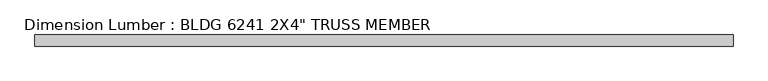
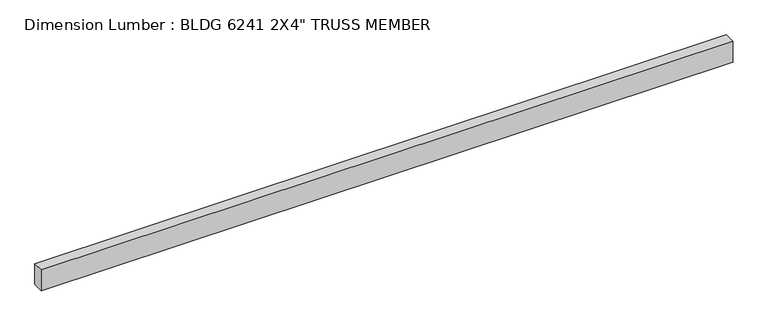
"""IFC4 building model written with IfcOpenShell, lengths in millimetres: beam geometry."""

from ifc_helpers import new_model, si_unit, frame, origin, place, context, project, spatial, polyline, outline, extrude, source, transform, mapped, element, save


def beam_6a2c9f8f(model_context):
    return source(origin(), model_context, "Body", "SweptSolid", [
        extrude(outline(polyline([(1599.9543138, 25.4), (1599.9543138, -25.4), (-1584.2465686, -25.4), (-1584.2465686, 25.4), (1599.9543138, 25.4)])), frame((0.0, 0.0, -50.8), z_axis=(0.0, 0.0, 1.0), x_axis=(1.0, 0.0, 0.0)), (0.0, 0.0, 1.0), 101.6),
    ])


if __name__ == "__main__":
    model = new_model("IFC4")
    model_context = context("Model", 3, world=origin())
    ifc_project = project(units=[si_unit("LENGTHUNIT", "METRE", prefix="MILLI")], contexts=[model_context])
    site = spatial("IfcSite", under=ifc_project)
    building = spatial("IfcBuilding", under=site)
    placement = place(None, origin())
    beam_shape = beam_6a2c9f8f(model_context)
    element("IfcBeam", 1, ObjectType="Dimension Lumber : BLDG 6241 2X4\" TRUSS MEMBER", at=placement, inside=building, context=model_context, shape_type="MappedRepresentation", body=[
        mapped(beam_shape, transform((0.0, 0.0, 0.0), x_axis=(1.0, 0.0, 0.0), y_axis=(0.0, 1.0, 0.0), z_axis=(0.0, 0.0, 1.0))),
    ])
    save(model, "model.ifc")

# Revit data of these elements
# Type "Dimension Lumber : BLDG 6241 2X4\" TRUSS MEMBER"
#   Assembly Code = "B10"
#   A = 0.273472 SF
#   Length [instance default] = 5' - 0"
#   b = 0' - 2"
#   d = 0' - 4"
#   Structural Material [instance default] = Softwood, Lumber
# Element 1 (IfcBeam, "Dimension Lumber : BLDG 6241 2X4\" TRUSS MEMBER")
#   Materials on its faces: "Softwood, Lumber"
# Materials
#   "Softwood, Lumber": class "Wood", colour RGB 223 192 134, transparency 0, Description = "Pinus Echinata", Cost = 0
